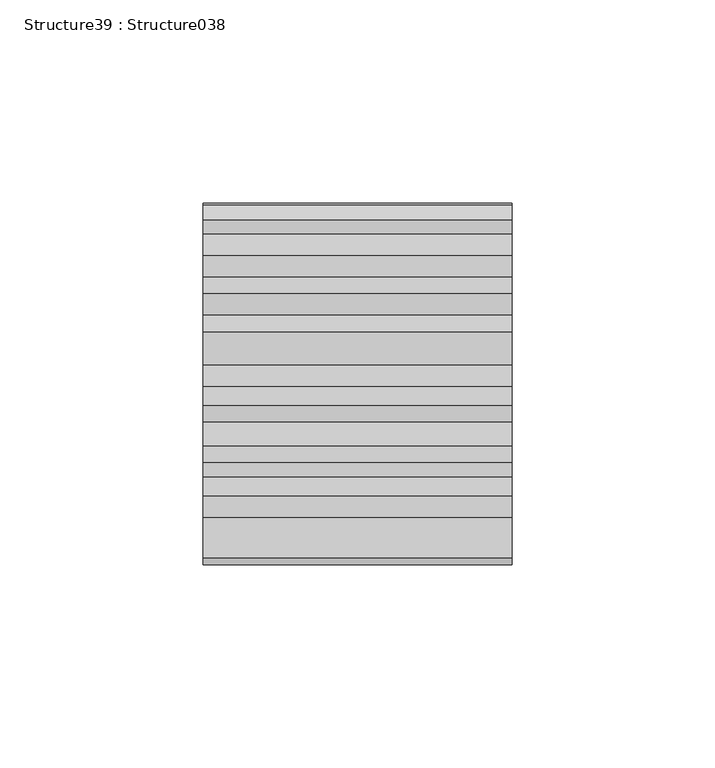
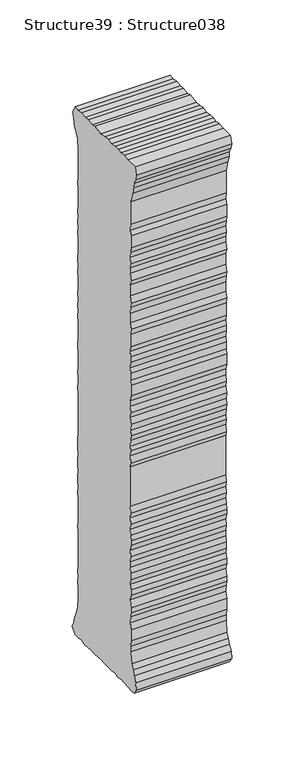
"""IFC4 building model written with IfcOpenShell, lengths in millimetres: proxy geometry, Structure39 : Structure038."""

from ifc_helpers import new_model, si_unit, frame, origin, place, context, project, spatial, polyline, outline, extrude, source, transform, mapped, element, save


def structure39_structure038_35b3715f(model_context):
    return source(origin(), model_context, "Body", "SweptSolid", [
        extrude(outline(polyline([(253757.0416964, 3575.6853037), (253758.7907153, 3569.8268927), (253761.1414609, 3565.1254015), (253762.3080083, 3559.8671125), (253764.6587539, 3555.1848766), (253760.5589894, 3550.4833855), (253756.4479927, 3550.4833855), (253751.1736577, 3551.6675836), (253747.6563647, 3550.4833855), (253742.3900527, 3550.4833855), (253737.7062122, 3551.0658569), (253733.5968201, 3550.4833855), (253728.9145842, 3551.0658569), (253724.8051921, 3551.6675836), (253720.1293745, 3551.0658569), (253709.5694724, 3551.0658569), (253704.8936549, 3551.6675836), (253701.3779664, 3550.4833855), (253696.1020268, 3551.6675836), (253692.5847338, 3551.0658569), (253686.7166951, 3551.0658569), (253682.0424822, 3550.4833855), (253678.5251892, 3551.0658569), (253675.5919722, 3555.1848766), (253676.1760482, 3561.025637), (253678.5251892, 3565.7094775), (253680.2742081, 3569.8268927), (253682.0424822, 3573.9266571), (253683.2090297, 3583.2863152), (253683.2090297, 3587.9685511), (253682.6249537, 3592.6700423), (253682.6249537, 3602.0280957), (253683.7931057, 3607.3393366), (253683.2090297, 3612.5976255), (253682.6249537, 3616.69739), (253682.6249537, 3620.7971545), (253683.7931057, 3626.6571701), (253682.6249537, 3631.3410106), (253682.6249537, 3636.0408972), (253683.7931057, 3640.114988), (253683.2090297, 3644.2420307), (253683.2090297, 3649.5003197), (253683.7931057, 3654.1841602), (253683.7931057, 3658.8840468), (253683.2090297, 3663.5598643), (253683.7931057, 3668.8261762), (253682.6249537, 3673.5276674), (253682.6249537, 3677.6274319), (253683.2090297, 3681.7271964), (253683.7931057, 3686.4030139), (253683.2090297, 3691.0868544), (253683.7931057, 3696.3884676), (253683.2090297, 3700.4705815), (253683.7931057, 3705.7545441), (253683.7931057, 3739.1592005), (253683.2090297, 3742.6748889), (253683.7931057, 3748.5429276), (253683.2090297, 3753.2171405), (253683.7931057, 3756.7440611), (253683.2090297, 3762.0023501), (253682.6249537, 3766.1021146), (253683.2090297, 3770.8036057), (253682.6249537, 3776.0618947), (253683.7931057, 3781.3282066), (253683.2090297, 3785.4456218), (253683.7931057, 3790.7039107), (253683.7931057, 3795.4037973), (253682.6249537, 3800.0876378), (253682.6249537, 3808.8888934), (253683.2090297, 3812.9726119), (253683.2090297, 3818.8310229), (253683.7931057, 3822.932392), (253683.2090297, 3828.2163546), (253683.2090297, 3832.8921721), (253683.7931057, 3836.9919366), (253683.2090297, 3841.0900965), (253683.2090297, 3851.6612309), (253682.6249537, 3856.3161885), (253683.7931057, 3861.0192843), (253683.7931057, 3869.2444869), (253683.2090297, 3874.5043805), (253682.6249537, 3878.5784713), (253683.7931057, 3883.8881076), (253683.7931057, 3893.246161), (253682.6249537, 3897.3475301), (253683.7931057, 3903.2059411), (253683.7931057, 3907.888177), (253683.2090297, 3911.4054701), (253683.7931057, 3916.6653636), (253683.2090297, 3921.3748778), (253682.6249537, 3925.4746423), (253682.6249537, 3935.4328178), (253683.7931057, 3939.5325823), (253683.2090297, 3944.8165449), (253683.2090297, 3964.1343784), (253680.8679117, 3972.3627903), (253679.0996376, 3978.2035506), (253678.5251892, 3982.3225704), (253676.7585196, 3986.4046842), (253675.5919722, 3991.0788971), (253677.3506187, 3996.9645864), (253687.3103988, 3996.9645864), (253692.5847338, 3997.5486624), (253697.2765973, 3996.9645864), (253700.787472, 3997.5486624), (253704.8936549, 3997.5486624), (253710.7440429, 3996.390138), (253714.8454119, 3997.5486624), (253719.5388801, 3996.9645864), (253724.8051921, 3996.390138), (253733.012744, 3997.5486624), (253737.1125085, 3996.390138), (253742.3900527, 3997.5486624), (253746.4882126, 3996.9645864), (253751.7657568, 3997.5486624), (253757.0416964, 3996.390138), (253760.5589894, 3997.5486624), (253764.0666549, 3991.0788971), (253762.3080083, 3987.5792547), (253761.7143047, 3981.7208437), (253757.0416964, 3972.3627903), (253756.4479927, 3962.9774586), (253756.4479927, 3940.718385), (253757.0416964, 3935.4328178), (253755.8655213, 3931.3346579), (253755.8655213, 3916.0909152), (253757.0416964, 3911.4054701), (253756.4479927, 3906.7328618), (253757.0416964, 3902.6314927), (253756.4479927, 3897.3475301), (253757.0416964, 3893.246161), (253756.4479927, 3888.5623205), (253755.8655213, 3884.4609514), (253755.8655213, 3879.7610648), (253757.0416964, 3870.4030114), (253756.4479927, 3865.1190488), (253757.0416964, 3859.8591552), (253755.8655213, 3855.7353217), (253755.8655213, 3845.8012153), (253757.0416964, 3842.2758992), (253756.4479927, 3836.4174882), (253757.0416964, 3831.732043), (253755.8655213, 3827.6162325), (253757.0416964, 3822.932392), (253756.4479927, 3817.6741031), (253756.4479927, 3813.5743386), (253755.8655213, 3808.8888934), (253755.8655213, 3804.1890069), (253757.0416964, 3798.9050443), (253755.8655213, 3790.7039107), (253755.8655213, 3780.1616592), (253757.0416964, 3775.4874463), (253756.4479927, 3771.9605256), (253755.8655213, 3767.2590344), (253757.0416964, 3762.5848215), (253756.4479927, 3756.7440611), (253755.8655213, 3752.04257), (253755.8655213, 3747.3587295), (253756.4479927, 3742.6748889), (253755.8655213, 3737.9750024), (253755.8655213, 3733.2991849), (253756.4479927, 3728.5992983), (253755.8655213, 3723.9154578), (253757.0416964, 3719.2316172), (253757.0416964, 3711.0304837), (253756.4479927, 3705.7545441), (253757.0416964, 3701.6547796), (253757.0416964, 3696.3884676), (253755.8655213, 3692.2710525), (253757.0416964, 3687.0127636), (253757.0416964, 3682.3289231), (253756.4479927, 3678.2018803), (253757.0416964, 3673.5276674), (253755.8655213, 3668.2437048), (253756.4479927, 3664.1423357), (253755.8655213, 3659.4584952), (253756.4479927, 3654.7842823), (253756.4479927, 3648.9258713), (253757.0416964, 3644.8245022), (253756.4479927, 3640.114988), (253756.4479927, 3634.856699), (253755.8655213, 3631.3410106), (253755.8655213, 3620.7971545), (253756.4479927, 3617.2718384), (253756.4479927, 3611.4134274), (253757.0416964, 3606.7295868), (253756.4479927, 3602.0280957), (253757.0416964, 3598.5284533), (253756.4479927, 3592.6700423), (253756.4479927, 3583.8864372), (253757.0416964, 3575.6853037)])), frame((-38594.2176606, 0.0, 0.0), z_axis=(1.0, 0.0, 0.0), x_axis=(0.0, 1.0, 0.0)), (0.0, 0.0, 1.0), 76.2),
    ])


if __name__ == "__main__":
    model = new_model("IFC4")
    model_context = context("Model", 3, world=origin())
    ifc_project = project(units=[si_unit("LENGTHUNIT", "METRE", prefix="MILLI")], contexts=[model_context])
    site = spatial("IfcSite", under=ifc_project)
    building = spatial("IfcBuilding", under=site)
    placement = place(None, origin())
    structure39_structure038_shape = structure39_structure038_35b3715f(model_context)
    element("IfcBuildingElementProxy", 1, Name="Structure39 : Structure038", ObjectType="Structure39 : Structure038", at=placement, inside=building, context=model_context, shape_type="MappedRepresentation", body=[
        mapped(structure39_structure038_shape, transform((0.0, 0.0, 0.0), x_axis=(1.0, 0.0, 0.0), y_axis=(0.0, 1.0, 0.0), z_axis=(0.0, 0.0, 1.0))),
    ])
    save(model, "model.ifc")

# Revit data of these elements
# Type "Structure39 : Structure038"
#   NameOverride = "Structure038"
# Element 1 (IfcBuildingElementProxy, "Structure39 : Structure038")
#   Materials on its faces: "BRUSHED ALUM. LETTERING"
# Materials
#   "BRUSHED ALUM. LETTERING": class "Unassigned", colour RGB 169 181 186, transparency 0, Cost = 0
